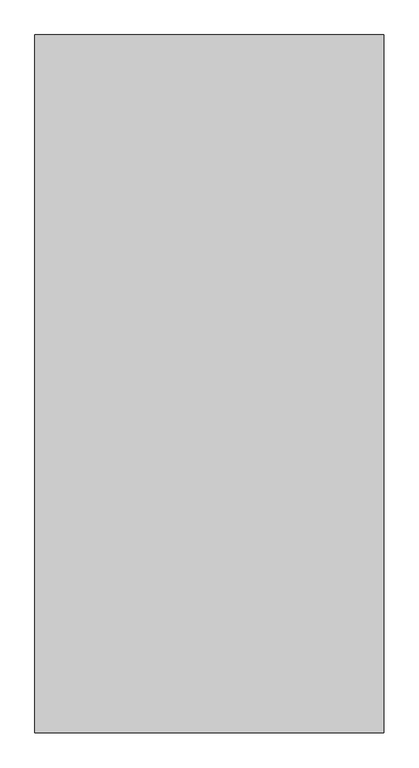
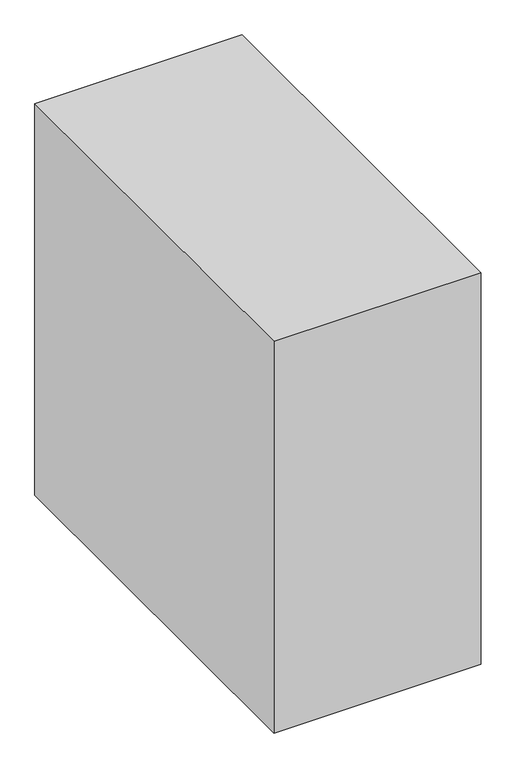
"""IFC4 building model written with IfcOpenShell, lengths in millimetres: proxy geometry, Space Planning Box_hec : Space Planning Box_hec."""

from ifc_helpers import new_model, si_unit, origin, origin_with_axes, place, context, project, spatial, polyline, outline, extrude, source, transform, mapped, element, save


def generic_models_542cc789(model_context):
    return source(origin(), model_context, "Body", "SweptSolid", [
        extrude(outline(polyline([(1500.0, 3000.0), (1500.0, -3000.0), (-1500.0, -3000.0), (-1500.0, 3000.0), (1500.0, 3000.0)])), origin_with_axes(), (0.0, 0.0, 1.0), 6000.0),
    ])


if __name__ == "__main__":
    model = new_model("IFC4")
    model_context = context("Model", 3, world=origin())
    ifc_project = project(units=[si_unit("LENGTHUNIT", "METRE", prefix="MILLI")], contexts=[model_context])
    site = spatial("IfcSite", under=ifc_project)
    building = spatial("IfcBuilding", under=site)
    placement = place(None, origin())
    generic_models_shape = generic_models_542cc789(model_context)
    element("IfcBuildingElementProxy", 1, Name="Space Planning Box_hec : Space Planning Box_hec", ObjectType="Space Planning Box_hec : Space Planning Box_hec", at=placement, inside=building, context=model_context, shape_type="MappedRepresentation", body=[
        mapped(generic_models_shape, transform((0.0, 0.0, 0.0), x_axis=(1.0, 0.0, 0.0), y_axis=(0.0, 1.0, 0.0), z_axis=(0.0, 0.0, 1.0))),
    ])
    save(model, "model.ifc")

# Revit data of these elements
# Type "Space Planning Box_hec : Space Planning Box_hec"
#   Type Comments = "..."
#   Room Name [instance default] = "?"
#   Interior Finish [instance default] = ""
#   Exterior Finish [instance default] = ""
#   Department [instance default] = ""
#   Assembly Code = "..."
#   Width [instance default] = 1524 mm
#   Program Area [instance default] = 0 m²
#   Length [instance default] = 1524 mm
#   Height [instance default] = 1524 mm
#   Area [instance default] = 2.32258 m²
#   Fill Color [instance default] = Cyan
#   Default Elevation = 0
# Element 1 (IfcBuildingElementProxy, "Space Planning Box_hec : Space Planning Box_hec")
#   Room Name = "LOTO Office Room"
#   Interior Finish = "IF2-1"
#   Exterior Finish = "EF1"
#   Department = "AR"
#   Width = 3000 mm
#   Program Area = 31.5 m²
#   Length = 6000 mm
#   Height = 6000 mm
#   Area = 18 m²
#   Fill Color = Lavender
#   Materials on its faces: "Lavender"
# Materials
#   "Cyan": class "Generic", colour RGB 0 255 255, transparency 0.2, Cost = 0
#   "Lavender": class "Generic", colour RGB 186 85 211, transparency 0.2, Cost = 0
